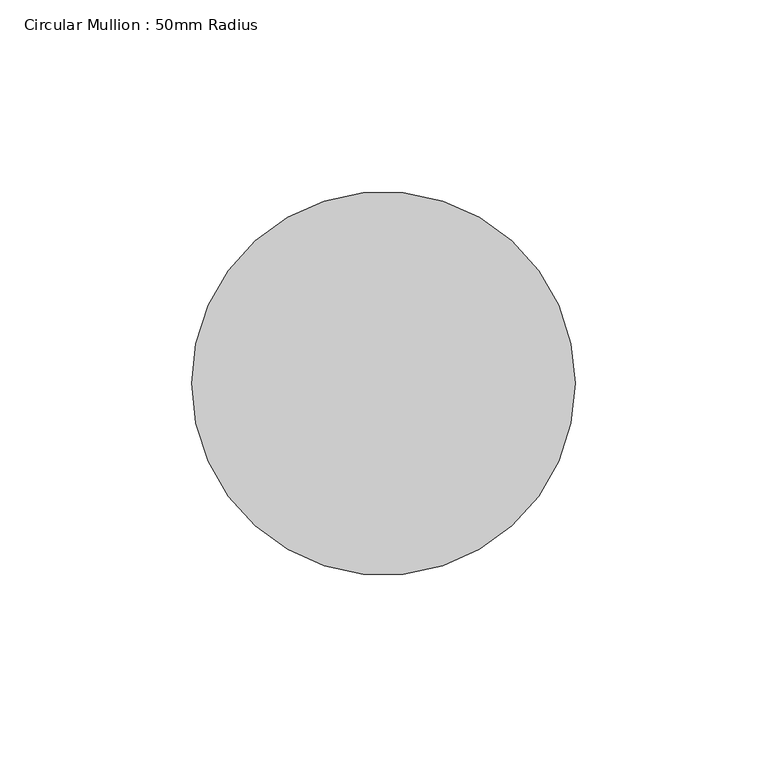
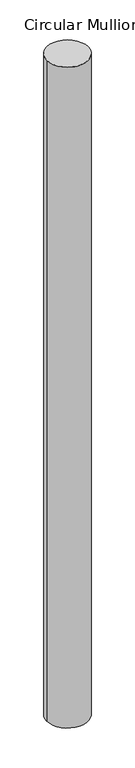
"""IFC4 building model written with IfcOpenShell, lengths in millimetres: member geometry, Circular Mullion : 50mm Radius."""

from ifc_helpers import new_model, si_unit, point, frame, origin, origin_2d, place, context, project, spatial, circle_curve, trimmed, segment, composite_curve, outline, extrude, source, transform, mapped, element, save


def circular_mullion_50mm_radius_4dfd7362(model_context):
    return source(origin(), model_context, "Body", "SweptSolid", [
        extrude(outline(composite_curve([segment(trimmed(circle_curve(origin_2d(), 50.0), [point((50.0, 0.0))], [point((-50.0, 0.0))], False, "CARTESIAN"), True, "CONTINUOUS"), segment(trimmed(circle_curve(origin_2d(), 50.0), [point((-50.0, 0.0))], [point((50.0, 0.0))], False, "CARTESIAN"), True, "CONTINUOUS")], self_intersect=False)), frame((0.0, 0.0, -1692.2662247), z_axis=(0.0, 0.0, 1.0), x_axis=(1.0, 0.0, 0.0)), (0.0, 0.0, 1.0), 1692.2662247),
    ])


if __name__ == "__main__":
    model = new_model("IFC4")
    model_context = context("Model", 3, world=origin())
    ifc_project = project(units=[si_unit("LENGTHUNIT", "METRE", prefix="MILLI")], contexts=[model_context])
    site = spatial("IfcSite", under=ifc_project)
    building = spatial("IfcBuilding", under=site)
    placement = place(None, origin())
    circular_mullion_50mm_radius_shape = circular_mullion_50mm_radius_4dfd7362(model_context)
    element("IfcMember", 1, ObjectType="Circular Mullion : 50mm Radius", at=placement, inside=building, context=model_context, shape_type="MappedRepresentation", body=[
        mapped(circular_mullion_50mm_radius_shape, transform((0.0, 0.0, 0.0), x_axis=(1.0, 0.0, 0.0), y_axis=(0.0, 1.0, 0.0), z_axis=(0.0, 0.0, 1.0))),
    ])
    save(model, "model.ifc")

# Revit data of these elements
# Type "Circular Mullion : 50mm Radius"
#   built-in parameter 1007350 = 0.164042 (stored number, unit not read)
# Element 1 (IfcMember, "Circular Mullion : 50mm Radius")
#   Materials on its faces: "Aluminium"
# Materials
#   "Aluminium": class "Metal", colour RGB 247 247 247, transparency 0, Description = "Aluminium 6061", Cost = 0
